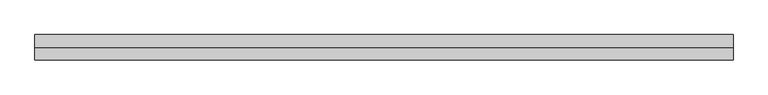
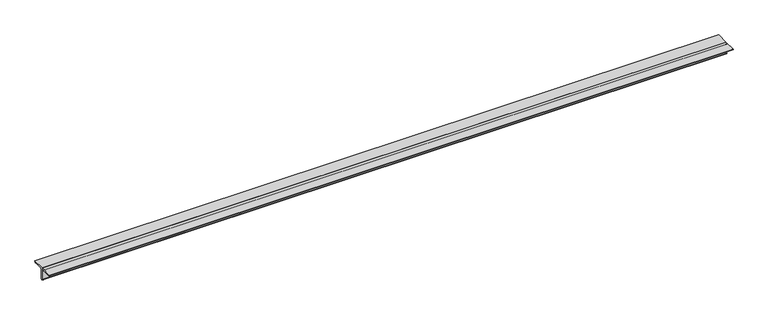
"""IFC4 building model written with IfcOpenShell, lengths in millimetres: member geometry, Steel Framing_2Ls_KS : H_SB_AR_S02_2Ls-100x100x10_VBR1."""

from ifc_helpers import new_model, si_unit, point, frame, frame_2d, origin, place, context, project, spatial, polyline, circle_curve, trimmed, segment, composite_curve, outline, extrude, source, transform, mapped, element, save


def member_ffdf4a1d(model_context):
    return source(origin(), model_context, "Body", "SweptSolid", [
        extrude(outline(composite_curve([segment(polyline([(0.0, 28.2), (100.0, 28.2)]), True, "CONTINUOUS"), segment(trimmed(circle_curve(frame_2d((90.0, 28.2)), 10.0), [point((100.0, 28.2))], [point((90.0, 18.2))], False, "CARTESIAN"), True, "CONTINUOUS"), segment(polyline([(90.0, 18.2), (20.0, 18.2)]), True, "CONTINUOUS"), segment(trimmed(circle_curve(frame_2d((20.0, 8.2)), 10.0), [point((20.0, 18.2))], [point((10.0, 8.2))], True, "CARTESIAN"), True, "CONTINUOUS"), segment(polyline([(10.0, 8.2), (10.0, -61.8)]), True, "CONTINUOUS"), segment(trimmed(circle_curve(frame_2d((0.0, -61.8)), 10.0), [point((10.0, -61.8))], [point((0.0, -71.8))], False, "CARTESIAN"), True, "CONTINUOUS"), segment(polyline([(0.0, -71.8), (0.0, 28.2)]), True, "CONTINUOUS")], self_intersect=False)), frame((-2590.3354834, 0.0, 0.0), z_axis=(1.0, 0.0, 0.0), x_axis=(0.0, 1.0, 0.0)), (0.0, 0.0, 1.0), 5505.8114308),
        extrude(outline(composite_curve([segment(polyline([(0.0, 28.2), (0.0, -71.8)]), True, "CONTINUOUS"), segment(trimmed(circle_curve(frame_2d((0.0, -61.8)), 10.0), [point((0.0, -71.8))], [point((-10.0, -61.8))], False, "CARTESIAN"), True, "CONTINUOUS"), segment(polyline([(-10.0, -61.8), (-10.0, 8.2)]), True, "CONTINUOUS"), segment(trimmed(circle_curve(frame_2d((-20.0, 8.2)), 10.0), [point((-10.0, 8.2))], [point((-20.0, 18.2))], True, "CARTESIAN"), True, "CONTINUOUS"), segment(polyline([(-20.0, 18.2), (-90.0, 18.2)]), True, "CONTINUOUS"), segment(trimmed(circle_curve(frame_2d((-90.0, 28.2)), 10.0), [point((-90.0, 18.2))], [point((-100.0, 28.2))], False, "CARTESIAN"), True, "CONTINUOUS"), segment(polyline([(-100.0, 28.2), (0.0, 28.2)]), True, "CONTINUOUS")], self_intersect=False)), frame((-2590.3354834, 0.0, 0.0), z_axis=(1.0, 0.0, 0.0), x_axis=(0.0, 1.0, 0.0)), (0.0, 0.0, 1.0), 5505.8114308),
    ])


if __name__ == "__main__":
    model = new_model("IFC4")
    model_context = context("Model", 3, world=origin())
    ifc_project = project(units=[si_unit("LENGTHUNIT", "METRE", prefix="MILLI")], contexts=[model_context])
    site = spatial("IfcSite", under=ifc_project)
    building = spatial("IfcBuilding", under=site)
    placement = place(None, origin())
    member_shape = member_ffdf4a1d(model_context)
    element("IfcMember", 1, ObjectType="Steel Framing_2Ls_KS : H_SB_AR_S02_2Ls-100x100x10_VBR1", at=placement, inside=building, context=model_context, shape_type="MappedRepresentation", body=[
        mapped(member_shape, transform((0.0, 0.0, 0.0), x_axis=(1.0, 0.0, 0.0), y_axis=(0.0, 1.0, 0.0), z_axis=(0.0, 0.0, 1.0))),
    ])
    save(model, "model.ifc")

# Revit data of these elements
# Type "Steel Framing_2Ls_KS : H_SB_AR_S02_2Ls-100x100x10_VBR1"
#   Type Comments = "MAIN"
#   Type Mark = "VBR1"
#   H_SectionID = "2Ls-100x100x10"
#   Assembly Code = "B10"
#   Legs = "LLBB"
#   H_Ratio for Additional Steel Plate = 0.2
#   W = 0
#   Perimeter = 0.80 m²/m
#   Nominal Weight = 29.80 kgf/m
#   Length [instance default] = 1524 mm
#   Space = 0 mm
#   b = 100 mm
#   d = 100 mm
#   t = 10 mm
#   y = 28.2 mm
#   A = 0.0038 m²
#   Structural Material [instance default] = Steel, 45-345
# Element 1 (IfcMember, "Steel Framing_2Ls_KS : H_SB_AR_S02_2Ls-100x100x10_VBR1")
#   Materials on its faces: "Steel, 45-345"
# Materials
#   "Steel, 45-345": class "Metal", colour RGB 189 187 185, transparency 0, Description = "Steel 345 MPa", Cost = 0
